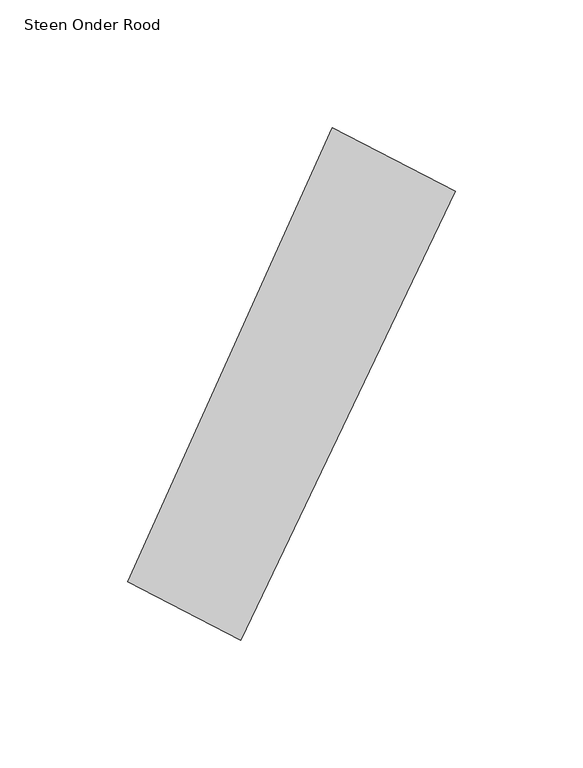
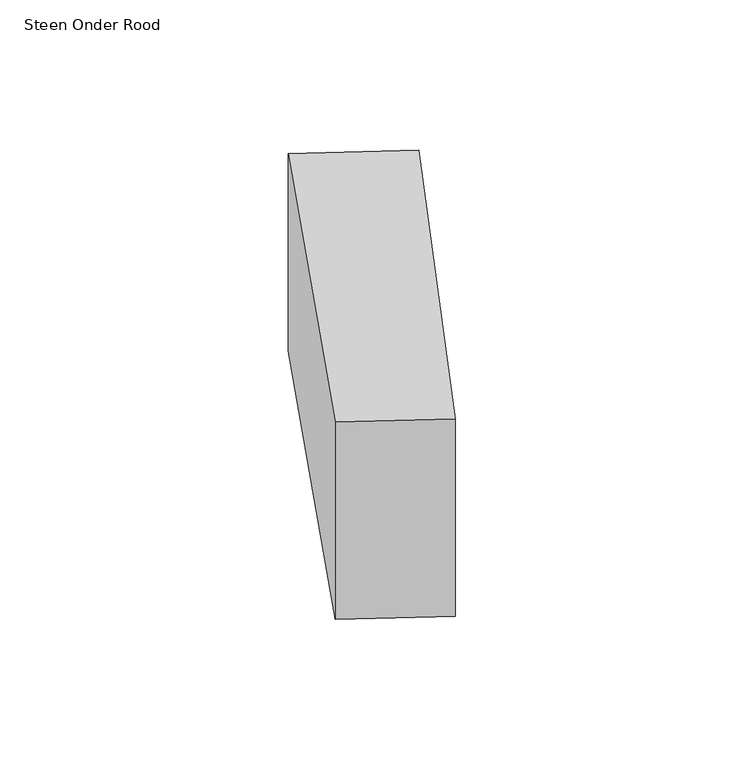
"""IFC4 building model written with IfcOpenShell, lengths in millimetres: proxy geometry, 00_GMA_steen_versie_4 : Steen Onder Rood."""

import ifcopenshell
import ifcopenshell.guid

model = None  # the IFC model being written
_history = None  # IfcOwnerHistory: only IFC2X3 demands one
_inside = {}  # id of a spatial element -> (the spatial element, [elements in it])
_under = {}  # id of a project, library or spatial element -> (it, [spatial elements below it])
_declared = {}  # id of a project -> (the project, [libraries it declares])
_typed = {}  # id of a type object -> (the type object, [elements of that type])
_made_of = {}  # id of a material, layer set ... -> (it, [elements and type objects made of it])


def new_model(schema):
    """Start an empty IFC model of exactly this schema.

    Asked for "IFC4X3", IfcOpenShell would pick the latest addendum, in which some entities
    have other attributes; the version numbers below select the first issue.
    IFC2X3 requires an IfcOwnerHistory on every rooted entity: one is made here for all.
    """
    global model, _history
    if schema == "IFC4X3":
        model = ifcopenshell.file(schema_version=(4, 3, 0, 0))
    else:
        model = ifcopenshell.file(schema=schema)
    _inside.clear()
    _under.clear()
    _declared.clear()
    _typed.clear()
    _made_of.clear()
    _history = None
    if model.schema == "IFC2X3":
        org = make("IfcOrganization", Name="unknown")
        user = make(
            "IfcPersonAndOrganization",
            ThePerson=make("IfcPerson", FamilyName="unknown"),
            TheOrganization=org,
        )
        app = make(
            "IfcApplication",
            ApplicationDeveloper=org,
            Version="unknown",
            ApplicationFullName="unknown",
            ApplicationIdentifier="unknown",
        )
        _history = make(
            "IfcOwnerHistory",
            OwningUser=user,
            OwningApplication=app,
            ChangeAction="ADDED",
            CreationDate=0,
        )
    return model


def make(cls, **values):
    """One entity of the class cls with the attributes given. An attribute that is None is left unset."""
    return model.create_entity(
        cls, **{name: value for name, value in values.items() if value is not None}
    )


def rooted(cls, **values):
    """An entity with a GlobalId (a new one), such as an element, a storey or a relation."""
    return make(cls, GlobalId=ifcopenshell.guid.new(), OwnerHistory=_history, **values)


def si_unit(unit_type, name, prefix=None):
    """IfcSIUnit, for example si_unit("LENGTHUNIT", "METRE", prefix="MILLI")."""
    return make("IfcSIUnit", UnitType=unit_type, Prefix=prefix, Name=name)


def assignment(units):
    """IfcUnitAssignment: the units of a project."""
    return None if units is None else make("IfcUnitAssignment", Units=units)


def point(xyz):
    """IfcCartesianPoint."""
    return None if xyz is None else make("IfcCartesianPoint", Coordinates=xyz)


def direction(xyz):
    """IfcDirection."""
    return None if xyz is None else make("IfcDirection", DirectionRatios=xyz)


def frame(location, z_axis=None, x_axis=None):
    """IfcAxis2Placement3D, a coordinate frame: its origin and axes. An axis left out is left unset."""
    return make(
        "IfcAxis2Placement3D",
        Location=point(location),
        Axis=direction(z_axis),
        RefDirection=direction(x_axis),
    )


def origin():
    """The frame at (0, 0, 0) with its axes left unset."""
    return frame((0.0, 0.0, 0.0))


def origin_with_axes():
    """The frame at (0, 0, 0) with the z axis (0, 0, 1) and the x axis (1, 0, 0) written out."""
    return frame((0.0, 0.0, 0.0), z_axis=(0.0, 0.0, 1.0), x_axis=(1.0, 0.0, 0.0))


def place(relative_to, where):
    """IfcLocalPlacement: puts the frame where relative to a parent placement (None: the world)."""
    return make(
        "IfcLocalPlacement", PlacementRelTo=relative_to, RelativePlacement=where
    )


def context(
    kind, dimensions, precision=None, world=None, true_north=None, identifier=None
):
    """IfcGeometricRepresentationContext, for example the 3D "Model" context."""
    return make(
        "IfcGeometricRepresentationContext",
        ContextIdentifier=identifier,
        ContextType=kind,
        CoordinateSpaceDimension=dimensions,
        Precision=precision,
        WorldCoordinateSystem=world,
        TrueNorth=true_north,
    )


def project(units=None, contexts=None):
    """IfcProject with its units and contexts."""
    return rooted(
        "IfcProject",
        Name="project",
        RepresentationContexts=contexts,
        UnitsInContext=assignment(units),
    )


def spatial(cls, under=None, at=None, **own):
    """A site, building, storey or space (cls), placed at a placement, below another one or the project."""
    s = rooted(cls, ObjectPlacement=at, **own)
    if under is not None:
        _under.setdefault(under.id(), (under, []))[1].append(s)
    return s


def polyline(points):
    """IfcPolyline through the points."""
    return make("IfcPolyline", Points=[point(p) for p in points])


def outline(outer, holes=None, kind="AREA"):
    """IfcArbitraryClosedProfileDef: a profile drawn as a closed curve; with holes, ...WithVoids."""
    if holes is None:
        return make("IfcArbitraryClosedProfileDef", ProfileType=kind, OuterCurve=outer)
    return make(
        "IfcArbitraryProfileDefWithVoids",
        ProfileType=kind,
        OuterCurve=outer,
        InnerCurves=holes,
    )


def extrude(swept, where, along, depth):
    """IfcExtrudedAreaSolid: the profile swept, set in the frame where, extruded along a direction by depth."""
    return make(
        "IfcExtrudedAreaSolid",
        SweptArea=swept,
        Position=where,
        ExtrudedDirection=direction(along),
        Depth=depth,
    )


def shape(context_of_items, identifier, shape_type, items):
    """IfcShapeRepresentation: the items that make up one representation, for example the "Body"."""
    return make(
        "IfcShapeRepresentation",
        ContextOfItems=context_of_items,
        RepresentationIdentifier=identifier,
        RepresentationType=shape_type,
        Items=items,
    )


def source(mapping_origin, context_of_items, identifier, shape_type, items):
    """IfcRepresentationMap: a shape defined once, which mapped items show again and again."""
    return make(
        "IfcRepresentationMap",
        MappingOrigin=mapping_origin,
        MappedRepresentation=shape(context_of_items, identifier, shape_type, items),
    )


def transform(
    local_origin,
    x_axis=None,
    y_axis=None,
    z_axis=None,
    scale=None,
    scale2=None,
    scale3=None,
    uniform=True,
):
    """IfcCartesianTransformationOperator3D, or its non-uniform kind. x_axis, y_axis, z_axis: its Axis1, 2, 3."""
    if uniform:
        return make(
            "IfcCartesianTransformationOperator3D",
            Axis1=direction(x_axis),
            Axis2=direction(y_axis),
            LocalOrigin=point(local_origin),
            Scale=scale,
            Axis3=direction(z_axis),
        )
    return make(
        "IfcCartesianTransformationOperator3DnonUniform",
        Axis1=direction(x_axis),
        Axis2=direction(y_axis),
        LocalOrigin=point(local_origin),
        Scale=scale,
        Axis3=direction(z_axis),
        Scale2=scale2,
        Scale3=scale3,
    )


def mapped(mapping_source, mapping_target):
    """IfcMappedItem: shows the shape of a source again, moved by a transform."""
    return make(
        "IfcMappedItem", MappingSource=mapping_source, MappingTarget=mapping_target
    )


def made_of(thing, what):
    """Note that an element or type object is made of a material, layer set ...; save() writes the relation."""
    if what is not None:
        _made_of.setdefault(what.id(), (what, []))[1].append(thing)
    return thing


def element(
    cls,
    number,
    at=None,
    inside=None,
    cuts=None,
    type_object=None,
    material=None,
    context=None,
    identifier="Body",
    shape_type=None,
    held_by="IfcProductDefinitionShape",
    body=None,
    shapes=None,
    **own,
):
    """One element of the class cls, such as IfcWall. Its Tag is "e" and its number.

    at: its placement. inside: the storey or other place that contains it. cuts: it is an
    opening in that element (IfcRelVoidsElement). A single representation is given by context,
    identifier, shape_type and body (its items); several are given by shapes. held_by: the class
    of the entity that holds the representations. save() writes the other relations.
    """
    e = rooted(cls, Tag="e%d" % number, ObjectPlacement=at, **own)
    if body is not None:
        shapes = [shape(context, identifier, shape_type, body)]
    if shapes is not None:
        e.Representation = make(held_by, Representations=shapes)
    if inside is not None:
        _inside.setdefault(inside.id(), (inside, []))[1].append(e)
    if cuts is not None:
        rooted(
            "IfcRelVoidsElement", RelatingBuildingElement=cuts, RelatedOpeningElement=e
        )
    if type_object is not None:
        _typed.setdefault(type_object.id(), (type_object, []))[1].append(e)
    return made_of(e, material)


def aggregate(whole, parts):
    """IfcRelAggregates: a whole, such as a stair, and the parts it consists of."""
    return rooted("IfcRelAggregates", RelatingObject=whole, RelatedObjects=parts)


def save(model, path):
    """Write the relations noted so far, then the file.

    IfcRelAggregates (storeys below a building ...), IfcRelContainedInSpatialStructure (elements
    in a storey), IfcRelDefinesByType, IfcRelAssociatesMaterial and IfcRelDeclares: one each for
    every whole, place, type object, material and project.
    """
    for whole, parts in _under.values():
        aggregate(whole, parts)
    for where, things in _inside.values():
        rooted(
            "IfcRelContainedInSpatialStructure",
            RelatedElements=things,
            RelatingStructure=where,
        )
    for kind, things in _typed.values():
        rooted("IfcRelDefinesByType", RelatedObjects=things, RelatingType=kind)
    for what, things in _made_of.values():
        rooted("IfcRelAssociatesMaterial", RelatedObjects=things, RelatingMaterial=what)
    for by, libraries in _declared.values():
        rooted("IfcRelDeclares", RelatingContext=by, RelatedDefinitions=libraries)
    model.write(path)


def steen_onder_rood_423ca539(model_context):
    return source(origin(), model_context, "Body", "SweptSolid", [
        extrude(outline(polyline([(142.0881793, 156.6728912), (57.988338, -19.3830646), (13.6146093, 3.6597694), (93.870346, 181.716615), (142.0881793, 156.6728912)])), origin_with_axes(), (0.0, 0.0, 1.0), 100.0),
    ])


if __name__ == "__main__":
    model = new_model("IFC4")
    model_context = context("Model", 3, world=origin())
    ifc_project = project(units=[si_unit("LENGTHUNIT", "METRE", prefix="MILLI")], contexts=[model_context])
    site = spatial("IfcSite", under=ifc_project)
    building = spatial("IfcBuilding", under=site)
    placement = place(None, origin())
    steen_onder_rood_shape = steen_onder_rood_423ca539(model_context)
    element("IfcBuildingElementProxy", 1, Name="00_GMA_steen_versie_4 : Steen Onder Rood", ObjectType="00_GMA_steen_versie_4 : Steen Onder Rood", at=placement, inside=building, context=model_context, shape_type="MappedRepresentation", body=[
        mapped(steen_onder_rood_shape, transform((0.0, 0.0, 0.0), x_axis=(1.0, 0.0, 0.0), y_axis=(0.0, 1.0, 0.0), z_axis=(0.0, 0.0, 1.0))),
    ])
    save(model, "model.ifc")

# Revit data of these elements
# Type "00_GMA_steen_versie_4 : Steen Onder Rood"
#   StootVoegHalfBoven [instance default] = 5 mm
#   StootVoegHalf [instance default] = 5 mm
#   StootVoegBreedteOnder = 10 mm
#   StootVoegBreedteBoven = 10 mm
#   Steendikte = 100 mm
#   LintVoegOnderHalf = 0 mm
#   LintVoegOnder = 0 mm
#   LintVoegBovenHalf = 5 mm
#   LintVoegBoven = 10 mm
#   materiaal = 21_steen_rood
#   MateriaalVoeg = none
#   Default Elevation = 0
# Element 1 (IfcBuildingElementProxy, "00_GMA_steen_versie_4 : Steen Onder Rood")
#   Materials on its faces: "21_steen_rood"
# Materials
#   "21_steen_rood": class "Unassigned", colour RGB 213 111 43, transparency 0, Cost = 0
